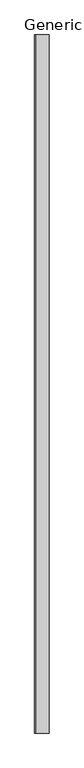
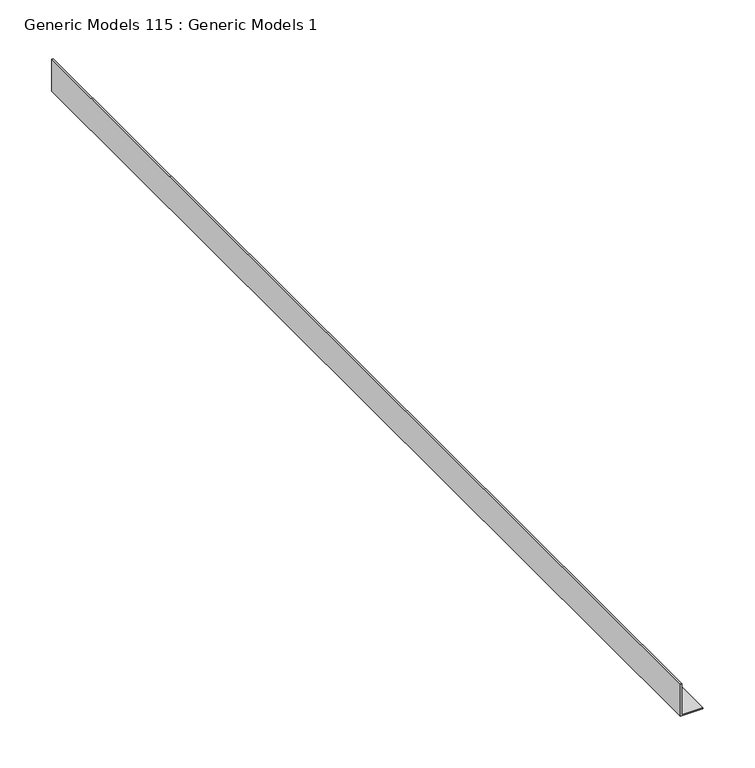
"""IFC4 building model written with IfcOpenShell, lengths in millimetres: proxy geometry, Generic Models 115 : Generic Models 1."""

from ifc_helpers import new_model, si_unit, frame, origin, place, context, project, spatial, polyline, outline, extrude, source, transform, mapped, element, save


def generic_models_115_generic_models_1_e8c90d4c(model_context):
    return source(origin(), model_context, "Body", "SweptSolid", [
        extrude(outline(polyline([(2277.1204978, 49799.875), (2239.0204978, 49799.875), (2239.0204978, 49825.275), (2240.6079978, 49825.275), (2240.6079978, 49801.4625), (2277.1204978, 49801.4625), (2277.1204978, 49799.875)])), frame((0.0, 0.0, 0.0), z_axis=(0.0, 1.0, 0.0), x_axis=(0.0, 0.0, 1.0)), (0.0, 0.0, 1.0), 1219.2),
    ])


if __name__ == "__main__":
    model = new_model("IFC4")
    model_context = context("Model", 3, world=origin())
    ifc_project = project(units=[si_unit("LENGTHUNIT", "METRE", prefix="MILLI")], contexts=[model_context])
    site = spatial("IfcSite", under=ifc_project)
    building = spatial("IfcBuilding", under=site)
    placement = place(None, origin())
    generic_models_115_generic_models_1_shape = generic_models_115_generic_models_1_e8c90d4c(model_context)
    element("IfcBuildingElementProxy", 1, Name="Generic Models 115 : Generic Models 1", ObjectType="Generic Models 115 : Generic Models 1", at=placement, inside=building, context=model_context, shape_type="MappedRepresentation", body=[
        mapped(generic_models_115_generic_models_1_shape, transform((0.0, 0.0, 0.0), x_axis=(1.0, 0.0, 0.0), y_axis=(0.0, 1.0, 0.0), z_axis=(0.0, 0.0, 1.0))),
    ])
    save(model, "model.ifc")

# Revit data of these elements
# Element 1 (IfcBuildingElementProxy, "Generic Models 115 : Generic Models 1")
#   Materials on its faces: "CEILING TRACK AS SCHEDULED"
# Materials
#   "CEILING TRACK AS SCHEDULED": class "Unassigned", colour RGB 210 209 208, transparency 0, Keynote = "M05121300.02", Cost = 0
